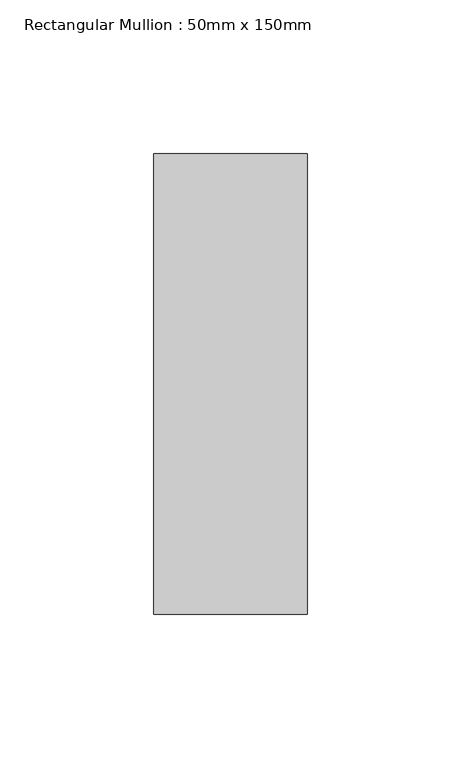
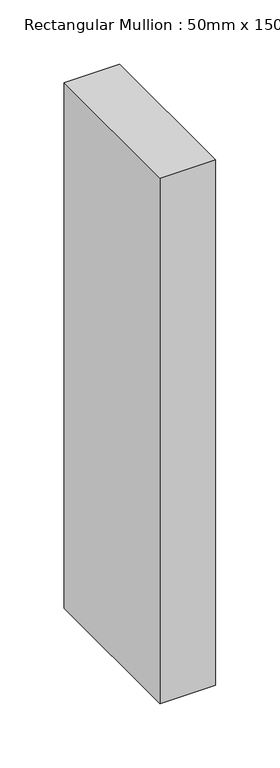
"""IFC4 building model written with IfcOpenShell, lengths in millimetres: member geometry, Rectangular Mullion : 50mm x 150mm."""

from ifc_helpers import new_model, si_unit, frame, origin, place, context, project, spatial, polyline, outline, extrude, source, transform, mapped, element, save


def rectangular_mullion_50mm_x_150mm_b3666dbd(model_context):
    return source(origin(), model_context, "Body", "SweptSolid", [
        extrude(outline(polyline([(0.0, 75.0), (0.0, -75.0), (-50.0, -75.0), (-50.0, 75.0), (0.0, 75.0)])), frame((0.0, 0.0, -500.0), z_axis=(0.0, 0.0, 1.0), x_axis=(1.0, 0.0, 0.0)), (0.0, 0.0, 1.0), 500.0),
    ])


if __name__ == "__main__":
    model = new_model("IFC4")
    model_context = context("Model", 3, world=origin())
    ifc_project = project(units=[si_unit("LENGTHUNIT", "METRE", prefix="MILLI")], contexts=[model_context])
    site = spatial("IfcSite", under=ifc_project)
    building = spatial("IfcBuilding", under=site)
    placement = place(None, origin())
    rectangular_mullion_50mm_x_150mm_shape = rectangular_mullion_50mm_x_150mm_b3666dbd(model_context)
    element("IfcMember", 1, ObjectType="Rectangular Mullion : 50mm x 150mm", at=placement, inside=building, context=model_context, shape_type="MappedRepresentation", body=[
        mapped(rectangular_mullion_50mm_x_150mm_shape, transform((0.0, 0.0, 0.0), x_axis=(1.0, 0.0, 0.0), y_axis=(0.0, 1.0, 0.0), z_axis=(0.0, 0.0, 1.0))),
    ])
    save(model, "model.ifc")

# Revit data of these elements
# Type "Rectangular Mullion : 50mm x 150mm"
#   built-in parameter 1007304 = 0.492126 (stored number, unit not read)
#   built-in parameter 1007301 = 0.082021 (stored number, unit not read)
#   built-in parameter 1007300 = 0.082021 (stored number, unit not read)
# Element 1 (IfcMember, "Rectangular Mullion : 50mm x 150mm")
#   Materials on its faces: "Aluminum"
# Materials
#   "Aluminum": class "Metal", colour RGB 244 244 244, transparency 0, Description = "Aluminum 6061", Cost = 0
